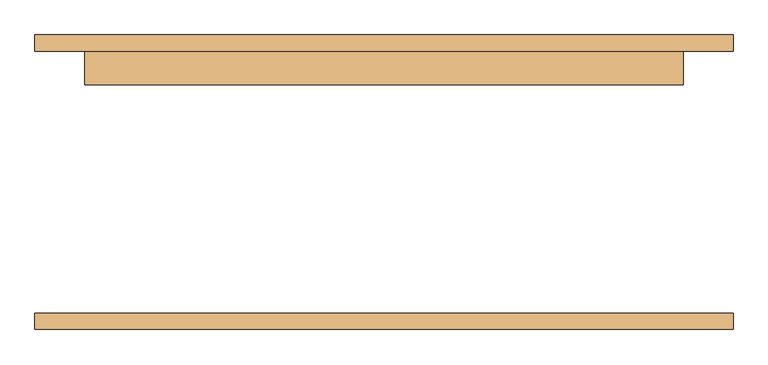
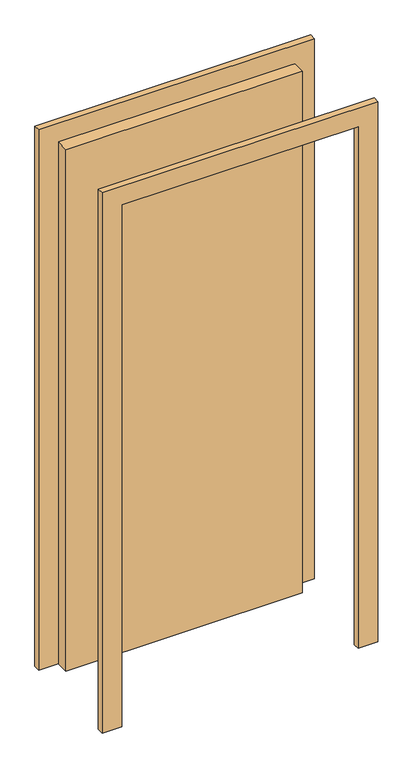
"""IFC4 building model written with IfcOpenShell, lengths in millimetres: door geometry, Одиночные-Щитовые : 0915 x 2134 мм."""

from ifc_helpers import new_model, si_unit, frame, origin, origin_with_axes, place, context, project, spatial, polyline, outline, extrude, source, transform, mapped, element, save


def door_d86ab3ce(model_context):
    return source(origin(), model_context, "Body", "SweptSolid", [
        extrude(outline(polyline([(2210.0, -533.5), (0.0, -533.5), (0.0, -457.5), (2134.0, -457.5), (2134.0, 457.5), (0.0, 457.5), (0.0, 533.5), (2210.0, 533.5), (2210.0, -533.5)])), frame((0.0, 200.0, 0.0), z_axis=(0.0, 1.0, 0.0), x_axis=(0.0, 0.0, 1.0)), (0.0, 0.0, 1.0), 25.0),
        extrude(outline(polyline([(2210.0, 533.5), (2210.0, -533.5), (0.0, -533.5), (0.0, -457.5), (2134.0, -457.5), (2134.0, 457.5), (0.0, 457.5), (0.0, 533.5), (2210.0, 533.5)])), frame((0.0, -225.0, 0.0), z_axis=(0.0, 1.0, 0.0), x_axis=(0.0, 0.0, 1.0)), (0.0, 0.0, 1.0), 25.0),
        extrude(outline(polyline([(457.5, 149.0), (-457.5, 149.0), (-457.5, 200.0), (457.5, 200.0), (457.5, 149.0)])), origin_with_axes(), (0.0, 0.0, 1.0), 2134.0),
    ])


if __name__ == "__main__":
    model = new_model("IFC4")
    model_context = context("Model", 3, world=origin())
    ifc_project = project(units=[si_unit("LENGTHUNIT", "METRE", prefix="MILLI")], contexts=[model_context])
    site = spatial("IfcSite", under=ifc_project)
    building = spatial("IfcBuilding", under=site)
    placement = place(None, origin())
    door_shape = door_d86ab3ce(model_context)
    element("IfcDoor", 1, ObjectType="Одиночные-Щитовые : 0915 x 2134 мм", at=placement, inside=building, context=model_context, shape_type="MappedRepresentation", body=[
        mapped(door_shape, transform((0.0, 0.0, 0.0), x_axis=(1.0, 0.0, 0.0), y_axis=(0.0, 1.0, 0.0), z_axis=(0.0, 0.0, 1.0))),
    ])
    save(model, "model.ifc")

# Revit data of these elements
# Type "Одиночные-Щитовые : 0915 x 2134 мм"
#   Type Mark = "20"
#   Construction Type Id = "MDOOR"
#   Analytic Construction = "Металл"
#   Thickness = 51 mm
#   Heat Transfer Coefficient (U) = 3.7021 W/(m²·K)
#   Height = 2134 mm
#   Проекционная подчистка-соединение наруж. = 25 mm
#   Проекционная подчистка-соединение внутр. = 25 mm
#   Проекционное соединение по ширине = 76 mm
#   Width = 915 mm
#   Материал двери = Дверь - Панель
#   Материал каркаса = Дверь - Каркас
#   Visual Light Transmittance = 0
#   Solar Heat Gain Coefficient = 0
#   Function = (empty or 0)
#   Wall Closure = (empty or 0)
# Element 1 (IfcDoor, "Одиночные-Щитовые : 0915 x 2134 мм")
#   Materials on its faces: "Дверь - Каркас", "Дверь - Панель"
# Materials
#   "Дверь - Панель": class "Древесина", colour RGB 210 159 95, transparency 0, Cost = 0
#   "Дверь - Каркас": class "Разное", colour RGB 118 70 51, transparency 0, Cost = 0
